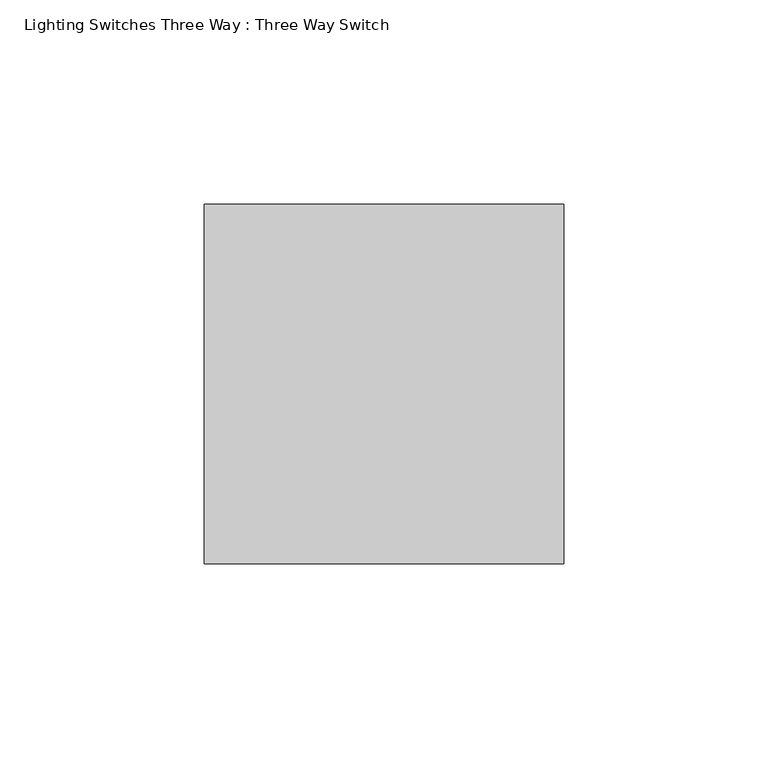
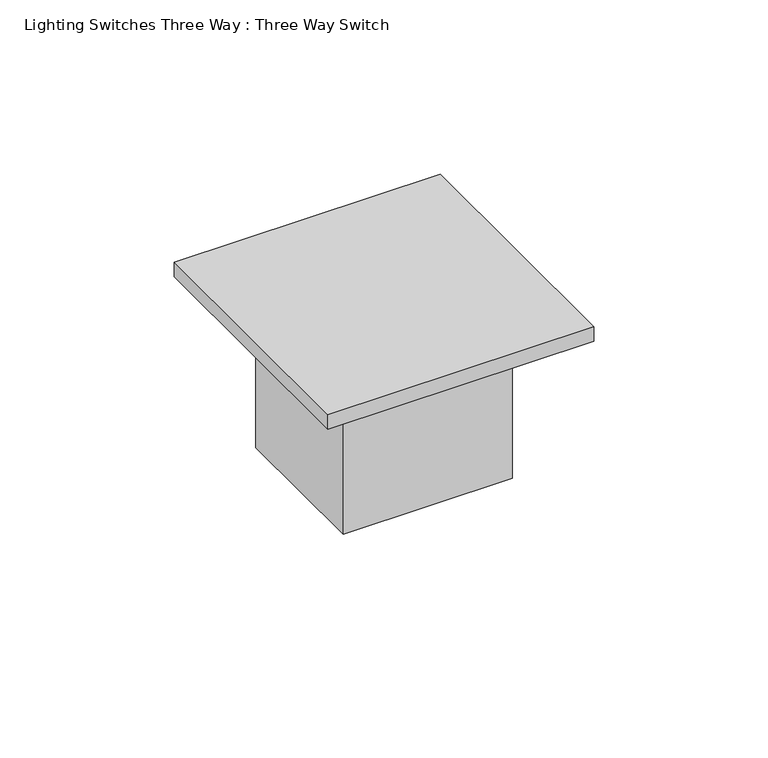
"""IFC4 building model written with IfcOpenShell, lengths in millimetres: switching device geometry, Lighting Switches Three Way : Three Way Switch."""

from ifc_helpers import new_model, si_unit, frame, origin, origin_with_axes, place, context, project, spatial, polyline, outline, extrude, source, transform, mapped, element, save


def lighting_switches_three_way_three_way_switch_4e4d8d92(model_context):
    return source(origin(), model_context, "Body", "SweptSolid", [
        extrude(outline(polyline([(44.0, -88.0), (-44.0, -88.0), (-44.0, 0.0), (44.0, 0.0), (44.0, -88.0)])), origin_with_axes(), (0.0, 0.0, 1.0), 5.0),
        extrude(outline(polyline([(28.0, -69.0), (-28.0, -69.0), (-28.0, -19.0), (28.0, -19.0), (28.0, -69.0)])), frame((0.0, 0.0, -54.0), z_axis=(0.0, 0.0, 1.0), x_axis=(1.0, 0.0, 0.0)), (0.0, 0.0, 1.0), 54.0),
    ])


if __name__ == "__main__":
    model = new_model("IFC4")
    model_context = context("Model", 3, world=origin())
    ifc_project = project(units=[si_unit("LENGTHUNIT", "METRE", prefix="MILLI")], contexts=[model_context])
    site = spatial("IfcSite", under=ifc_project)
    building = spatial("IfcBuilding", under=site)
    placement = place(None, origin())
    lighting_switches_three_way_three_way_switch_shape = lighting_switches_three_way_three_way_switch_4e4d8d92(model_context)
    element("IfcSwitchingDevice", 1, ObjectType="Lighting Switches Three Way : Three Way Switch", at=placement, inside=building, context=model_context, shape_type="MappedRepresentation", body=[
        mapped(lighting_switches_three_way_three_way_switch_shape, transform((0.0, 0.0, 0.0), x_axis=(1.0, 0.0, 0.0), y_axis=(0.0, 1.0, 0.0), z_axis=(0.0, 0.0, 1.0))),
    ])
    save(model, "model.ifc")

# Revit data of these elements
# Type "Lighting Switches Three Way : Three Way Switch"
#   Type Mark = "Lighting Switches Three Way"
#   Classification.MasterFormat.Number = ""
#   Classification.OmniClass.23.Number = "23-35 37 00"
#   Classification.OmniClass.23.Description = "Electrical Switches"
#   COBie.Type.CreatedBy = "info@mma.ie"
#   COBie.Type.CreatedOn = "2017-07-25T10:15:16"
#   COBie.Type.Name = "Lighting Switches Three Way"
#   COBie.Type.Category = "23-35 37 00 : Electrical Switches"
#   COBie.Type.Description = "Lighting Switches Three Way_Three Way Switch"
#   COBie.Type.AssetType = "Fixed"
#   COBie.Type.Manufacturer = ""
#   COBie.Type.ModelNumber = ""
#   Label = "3"
#   Keynote = "26 36 13.C"
#   COBie.Type.ReplacementCost = 0
#   Width = 88 mm
#   Switch Voltage [instance default] = 230 V
#   Lenght = 88 mm
#   Height = 59 mm
#   Default Elevation = 1200 mm
#   Apparent Load = 0 VA
#   3.W.S. Width = 88 mm
#   3.W.S. Height = 88 mm
#   3.W.S. Depth = 59 mm
#   COBie.Type = yes
#   Visibility 7 = no
#   Visibility 6 = no
#   Visibility 5 = no
#   Visibility 4 = yes
#   Visibility 3 = no
#   Visibility 2 = no
#   Visibility 1 = no
#   Ballast Number of Poles = 1
#   Load Classification = Other
#   3.W.S. Material = Metal - Chrome
# Materials
#   "Metal - Chrome": class "Metal", colour RGB 17 17 17, transparency 0, Comments = "Rendering appearance not upgraded "
